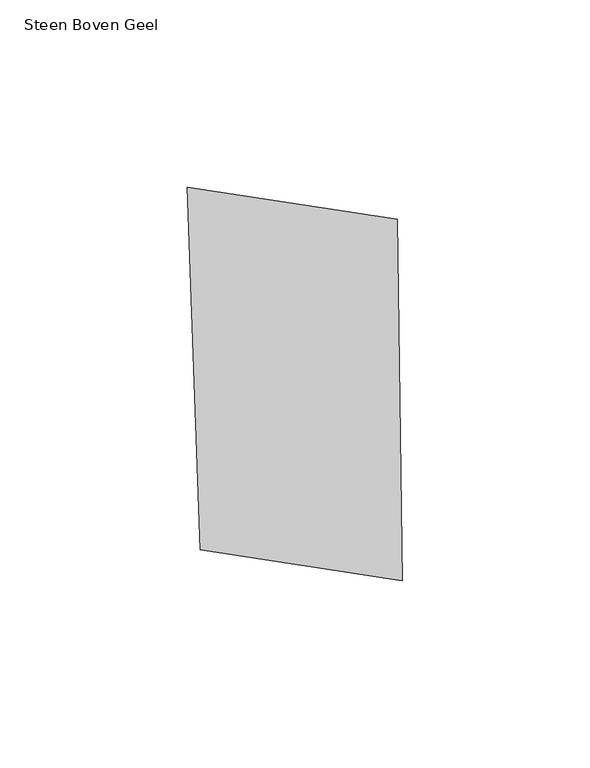
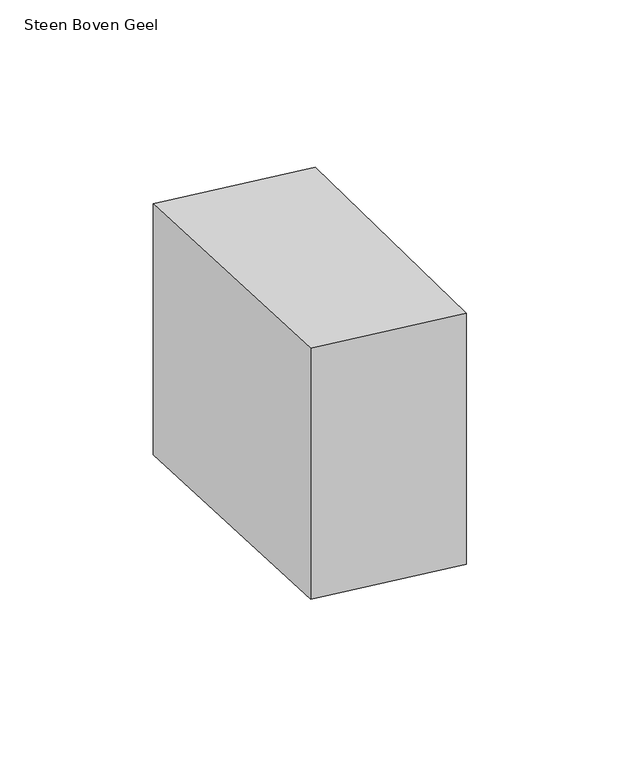
"""IFC4 building model written with IfcOpenShell, lengths in millimetres: proxy geometry, 00_GMA_steen_versie_4 : Steen Boven Geel."""

from ifc_helpers import new_model, si_unit, origin, origin_with_axes, place, context, project, spatial, polyline, outline, extrude, source, transform, mapped, element, save


def steen_boven_geel_d66ba735(model_context):
    return source(origin(), model_context, "Body", "SweptSolid", [
        extrude(outline(polyline([(99.9228464, 120.036338), (101.2300351, 23.6643873), (47.3026614, 31.8859382), (43.9059609, 128.5931858), (99.9228464, 120.036338)])), origin_with_axes(), (0.0, 0.0, 1.0), 100.0),
    ])


if __name__ == "__main__":
    model = new_model("IFC4")
    model_context = context("Model", 3, world=origin())
    ifc_project = project(units=[si_unit("LENGTHUNIT", "METRE", prefix="MILLI")], contexts=[model_context])
    site = spatial("IfcSite", under=ifc_project)
    building = spatial("IfcBuilding", under=site)
    placement = place(None, origin())
    steen_boven_geel_shape = steen_boven_geel_d66ba735(model_context)
    element("IfcBuildingElementProxy", 1, Name="00_GMA_steen_versie_4 : Steen Boven Geel", ObjectType="00_GMA_steen_versie_4 : Steen Boven Geel", at=placement, inside=building, context=model_context, shape_type="MappedRepresentation", body=[
        mapped(steen_boven_geel_shape, transform((0.0, 0.0, 0.0), x_axis=(1.0, 0.0, 0.0), y_axis=(0.0, 1.0, 0.0), z_axis=(0.0, 0.0, 1.0))),
    ])
    save(model, "model.ifc")

# Revit data of these elements
# Type "00_GMA_steen_versie_4 : Steen Boven Geel"
#   StootVoegHalfBoven [instance default] = 5 mm
#   StootVoegHalf [instance default] = 5 mm
#   StootVoegBreedteOnder = 10 mm
#   StootVoegBreedteBoven = 10 mm
#   Steendikte = 100 mm
#   LintVoegOnderHalf = 5 mm
#   LintVoegOnder = 10 mm
#   LintVoegBovenHalf = 0 mm
#   LintVoegBoven = 0 mm
#   materiaal = 21_steen_geel
#   MateriaalVoeg = none
#   Default Elevation = 0
# Element 1 (IfcBuildingElementProxy, "00_GMA_steen_versie_4 : Steen Boven Geel")
#   Materials on its faces: "21_steen_geel"
# Materials
#   "21_steen_geel": class "Unassigned", colour RGB 202 202 0, transparency 0, Cost = 0
